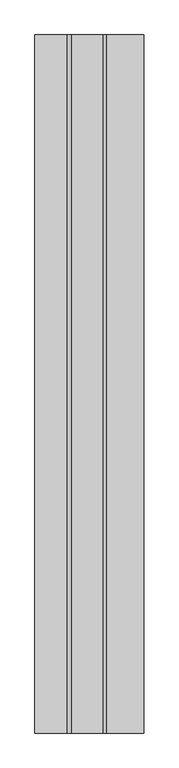
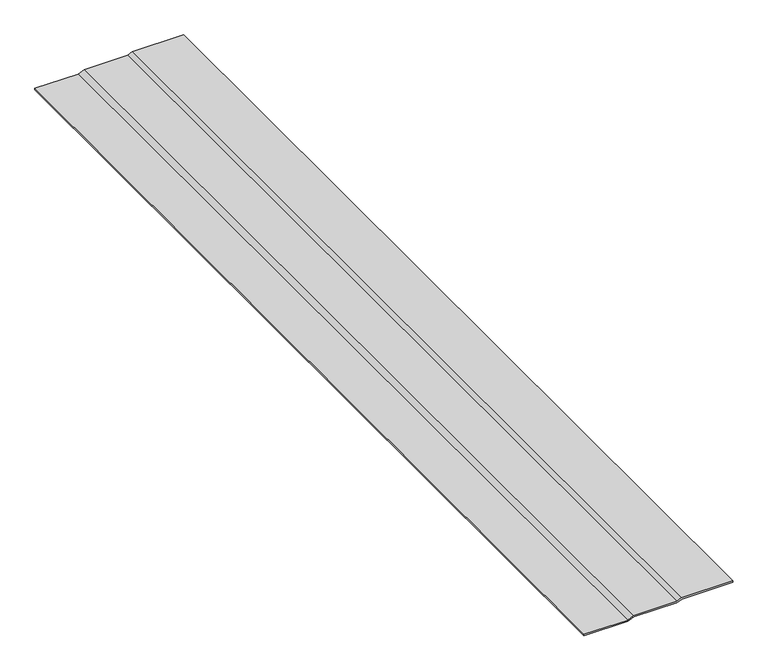
"""IFC4 building model written with IfcOpenShell, lengths in millimetres: proxy geometry, BITUMEN CAP SHEET4:BITUMEN CAP SHEET002:300114 : BITUMEN CAP SHEET4:BITUMEN CAP SHEET002:300114."""

import ifcopenshell
import ifcopenshell.guid

model = None  # the IFC model being written
_history = None  # IfcOwnerHistory: only IFC2X3 demands one
_inside = {}  # id of a spatial element -> (the spatial element, [elements in it])
_under = {}  # id of a project, library or spatial element -> (it, [spatial elements below it])
_declared = {}  # id of a project -> (the project, [libraries it declares])
_typed = {}  # id of a type object -> (the type object, [elements of that type])
_made_of = {}  # id of a material, layer set ... -> (it, [elements and type objects made of it])


def new_model(schema):
    """Start an empty IFC model of exactly this schema.

    Asked for "IFC4X3", IfcOpenShell would pick the latest addendum, in which some entities
    have other attributes; the version numbers below select the first issue.
    IFC2X3 requires an IfcOwnerHistory on every rooted entity: one is made here for all.
    """
    global model, _history
    if schema == "IFC4X3":
        model = ifcopenshell.file(schema_version=(4, 3, 0, 0))
    else:
        model = ifcopenshell.file(schema=schema)
    _inside.clear()
    _under.clear()
    _declared.clear()
    _typed.clear()
    _made_of.clear()
    _history = None
    if model.schema == "IFC2X3":
        org = make("IfcOrganization", Name="unknown")
        user = make(
            "IfcPersonAndOrganization",
            ThePerson=make("IfcPerson", FamilyName="unknown"),
            TheOrganization=org,
        )
        app = make(
            "IfcApplication",
            ApplicationDeveloper=org,
            Version="unknown",
            ApplicationFullName="unknown",
            ApplicationIdentifier="unknown",
        )
        _history = make(
            "IfcOwnerHistory",
            OwningUser=user,
            OwningApplication=app,
            ChangeAction="ADDED",
            CreationDate=0,
        )
    return model


def make(cls, **values):
    """One entity of the class cls with the attributes given. An attribute that is None is left unset."""
    return model.create_entity(
        cls, **{name: value for name, value in values.items() if value is not None}
    )


def rooted(cls, **values):
    """An entity with a GlobalId (a new one), such as an element, a storey or a relation."""
    return make(cls, GlobalId=ifcopenshell.guid.new(), OwnerHistory=_history, **values)


def si_unit(unit_type, name, prefix=None):
    """IfcSIUnit, for example si_unit("LENGTHUNIT", "METRE", prefix="MILLI")."""
    return make("IfcSIUnit", UnitType=unit_type, Prefix=prefix, Name=name)


def assignment(units):
    """IfcUnitAssignment: the units of a project."""
    return None if units is None else make("IfcUnitAssignment", Units=units)


def point(xyz):
    """IfcCartesianPoint."""
    return None if xyz is None else make("IfcCartesianPoint", Coordinates=xyz)


def direction(xyz):
    """IfcDirection."""
    return None if xyz is None else make("IfcDirection", DirectionRatios=xyz)


def frame(location, z_axis=None, x_axis=None):
    """IfcAxis2Placement3D, a coordinate frame: its origin and axes. An axis left out is left unset."""
    return make(
        "IfcAxis2Placement3D",
        Location=point(location),
        Axis=direction(z_axis),
        RefDirection=direction(x_axis),
    )


def origin():
    """The frame at (0, 0, 0) with its axes left unset."""
    return frame((0.0, 0.0, 0.0))


def place(relative_to, where):
    """IfcLocalPlacement: puts the frame where relative to a parent placement (None: the world)."""
    return make(
        "IfcLocalPlacement", PlacementRelTo=relative_to, RelativePlacement=where
    )


def context(
    kind, dimensions, precision=None, world=None, true_north=None, identifier=None
):
    """IfcGeometricRepresentationContext, for example the 3D "Model" context."""
    return make(
        "IfcGeometricRepresentationContext",
        ContextIdentifier=identifier,
        ContextType=kind,
        CoordinateSpaceDimension=dimensions,
        Precision=precision,
        WorldCoordinateSystem=world,
        TrueNorth=true_north,
    )


def project(units=None, contexts=None):
    """IfcProject with its units and contexts."""
    return rooted(
        "IfcProject",
        Name="project",
        RepresentationContexts=contexts,
        UnitsInContext=assignment(units),
    )


def spatial(cls, under=None, at=None, **own):
    """A site, building, storey or space (cls), placed at a placement, below another one or the project."""
    s = rooted(cls, ObjectPlacement=at, **own)
    if under is not None:
        _under.setdefault(under.id(), (under, []))[1].append(s)
    return s


def polyline(points):
    """IfcPolyline through the points."""
    return make("IfcPolyline", Points=[point(p) for p in points])


def outline(outer, holes=None, kind="AREA"):
    """IfcArbitraryClosedProfileDef: a profile drawn as a closed curve; with holes, ...WithVoids."""
    if holes is None:
        return make("IfcArbitraryClosedProfileDef", ProfileType=kind, OuterCurve=outer)
    return make(
        "IfcArbitraryProfileDefWithVoids",
        ProfileType=kind,
        OuterCurve=outer,
        InnerCurves=holes,
    )


def extrude(swept, where, along, depth):
    """IfcExtrudedAreaSolid: the profile swept, set in the frame where, extruded along a direction by depth."""
    return make(
        "IfcExtrudedAreaSolid",
        SweptArea=swept,
        Position=where,
        ExtrudedDirection=direction(along),
        Depth=depth,
    )


def shape(context_of_items, identifier, shape_type, items):
    """IfcShapeRepresentation: the items that make up one representation, for example the "Body"."""
    return make(
        "IfcShapeRepresentation",
        ContextOfItems=context_of_items,
        RepresentationIdentifier=identifier,
        RepresentationType=shape_type,
        Items=items,
    )


def source(mapping_origin, context_of_items, identifier, shape_type, items):
    """IfcRepresentationMap: a shape defined once, which mapped items show again and again."""
    return make(
        "IfcRepresentationMap",
        MappingOrigin=mapping_origin,
        MappedRepresentation=shape(context_of_items, identifier, shape_type, items),
    )


def transform(
    local_origin,
    x_axis=None,
    y_axis=None,
    z_axis=None,
    scale=None,
    scale2=None,
    scale3=None,
    uniform=True,
):
    """IfcCartesianTransformationOperator3D, or its non-uniform kind. x_axis, y_axis, z_axis: its Axis1, 2, 3."""
    if uniform:
        return make(
            "IfcCartesianTransformationOperator3D",
            Axis1=direction(x_axis),
            Axis2=direction(y_axis),
            LocalOrigin=point(local_origin),
            Scale=scale,
            Axis3=direction(z_axis),
        )
    return make(
        "IfcCartesianTransformationOperator3DnonUniform",
        Axis1=direction(x_axis),
        Axis2=direction(y_axis),
        LocalOrigin=point(local_origin),
        Scale=scale,
        Axis3=direction(z_axis),
        Scale2=scale2,
        Scale3=scale3,
    )


def mapped(mapping_source, mapping_target):
    """IfcMappedItem: shows the shape of a source again, moved by a transform."""
    return make(
        "IfcMappedItem", MappingSource=mapping_source, MappingTarget=mapping_target
    )


def made_of(thing, what):
    """Note that an element or type object is made of a material, layer set ...; save() writes the relation."""
    if what is not None:
        _made_of.setdefault(what.id(), (what, []))[1].append(thing)
    return thing


def element(
    cls,
    number,
    at=None,
    inside=None,
    cuts=None,
    type_object=None,
    material=None,
    context=None,
    identifier="Body",
    shape_type=None,
    held_by="IfcProductDefinitionShape",
    body=None,
    shapes=None,
    **own,
):
    """One element of the class cls, such as IfcWall. Its Tag is "e" and its number.

    at: its placement. inside: the storey or other place that contains it. cuts: it is an
    opening in that element (IfcRelVoidsElement). A single representation is given by context,
    identifier, shape_type and body (its items); several are given by shapes. held_by: the class
    of the entity that holds the representations. save() writes the other relations.
    """
    e = rooted(cls, Tag="e%d" % number, ObjectPlacement=at, **own)
    if body is not None:
        shapes = [shape(context, identifier, shape_type, body)]
    if shapes is not None:
        e.Representation = make(held_by, Representations=shapes)
    if inside is not None:
        _inside.setdefault(inside.id(), (inside, []))[1].append(e)
    if cuts is not None:
        rooted(
            "IfcRelVoidsElement", RelatingBuildingElement=cuts, RelatedOpeningElement=e
        )
    if type_object is not None:
        _typed.setdefault(type_object.id(), (type_object, []))[1].append(e)
    return made_of(e, material)


def aggregate(whole, parts):
    """IfcRelAggregates: a whole, such as a stair, and the parts it consists of."""
    return rooted("IfcRelAggregates", RelatingObject=whole, RelatedObjects=parts)


def save(model, path):
    """Write the relations noted so far, then the file.

    IfcRelAggregates (storeys below a building ...), IfcRelContainedInSpatialStructure (elements
    in a storey), IfcRelDefinesByType, IfcRelAssociatesMaterial and IfcRelDeclares: one each for
    every whole, place, type object, material and project.
    """
    for whole, parts in _under.values():
        aggregate(whole, parts)
    for where, things in _inside.values():
        rooted(
            "IfcRelContainedInSpatialStructure",
            RelatedElements=things,
            RelatingStructure=where,
        )
    for kind, things in _typed.values():
        rooted("IfcRelDefinesByType", RelatedObjects=things, RelatingType=kind)
    for what, things in _made_of.values():
        rooted("IfcRelAssociatesMaterial", RelatedObjects=things, RelatingMaterial=what)
    for by, libraries in _declared.values():
        rooted("IfcRelDeclares", RelatingContext=by, RelatedDefinitions=libraries)
    model.write(path)


def generic_models_ece583c1(model_context):
    return source(origin(), model_context, "Body", "SweptSolid", [
        extrude(outline(polyline([(40262.3752679, 77.2027316), (40259.2002678, 77.2027316), (40259.2002678, 169.3673932), (40264.4862773, 181.8322118), (40264.4862773, 272.546368), (40268.8188423, 282.2627545), (40268.8188423, 389.4739656), (40271.994072, 389.4739656), (40271.994072, 281.587469), (40267.6612773, 271.8705675), (40267.6612773, 181.1868119), (40262.3752679, 168.7219932), (40262.3752679, 77.2027316)])), frame((0.0, -774.5581163, 0.0), z_axis=(0.0, 1.0, 0.0), x_axis=(0.0, 0.0, 1.0)), (0.0, 0.0, 1.0), 2000.25),
    ])


if __name__ == "__main__":
    model = new_model("IFC4")
    model_context = context("Model", 3, world=origin())
    ifc_project = project(units=[si_unit("LENGTHUNIT", "METRE", prefix="MILLI")], contexts=[model_context])
    site = spatial("IfcSite", under=ifc_project)
    building = spatial("IfcBuilding", under=site)
    placement = place(None, origin())
    generic_models_shape = generic_models_ece583c1(model_context)
    element("IfcBuildingElementProxy", 1, Name="BITUMEN CAP SHEET4:BITUMEN CAP SHEET002:300114 : BITUMEN CAP SHEET4:BITUMEN CAP SHEET002:300114", ObjectType="BITUMEN CAP SHEET4:BITUMEN CAP SHEET002:300114 : BITUMEN CAP SHEET4:BITUMEN CAP SHEET002:300114", at=placement, inside=building, context=model_context, shape_type="MappedRepresentation", body=[
        mapped(generic_models_shape, transform((0.0, 0.0, 0.0), x_axis=(1.0, 0.0, 0.0), y_axis=(0.0, 1.0, 0.0), z_axis=(0.0, 0.0, 1.0))),
    ])
    save(model, "model.ifc")

# Revit data of these elements
# Type "BITUMEN CAP SHEET4:BITUMEN CAP SHEET002:300114 : BITUMEN CAP SHEET4:BITUMEN CAP SHEET002:300114"
#   NameOverride = "BITUMEN CAP SHEET4:BITUMEN CAP SHEET002:300114"
#   ObjectTypeOverride = "BITUMEN CAP SHEET4:BITUMEN CAP SHEET002"
#   Reference = "BITUMEN CAP SHEET002"
#   Category = "Generic Models"
#   Tag = "300114"
# Element 1 (IfcBuildingElementProxy, "BITUMEN CAP SHEET4:BITUMEN CAP SHEET002:300114 : BITUMEN CAP SHEET4:BITUMEN CAP SHEET002:300114")
#   Materials on its faces: "MODIFIED BITUMEN GRANULE SURFACED CAP SHEET"
# Materials
#   "MODIFIED BITUMEN GRANULE SURFACED CAP SHEET": class "Unassigned", colour RGB 85 85 127, transparency 0
